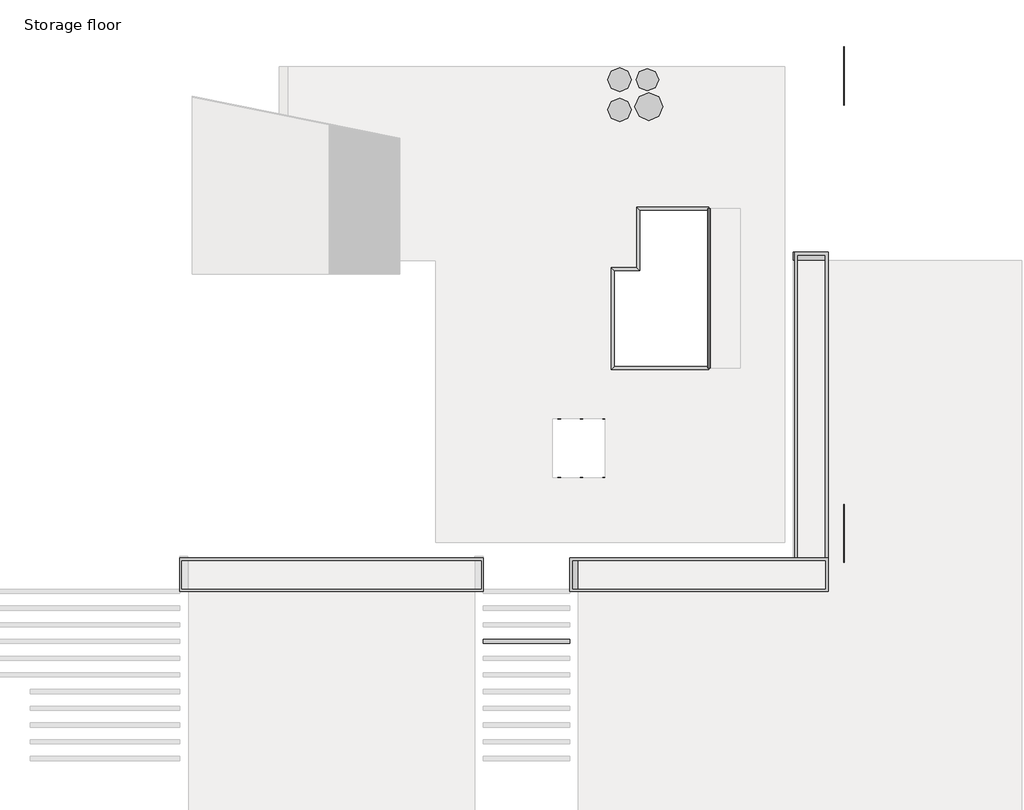
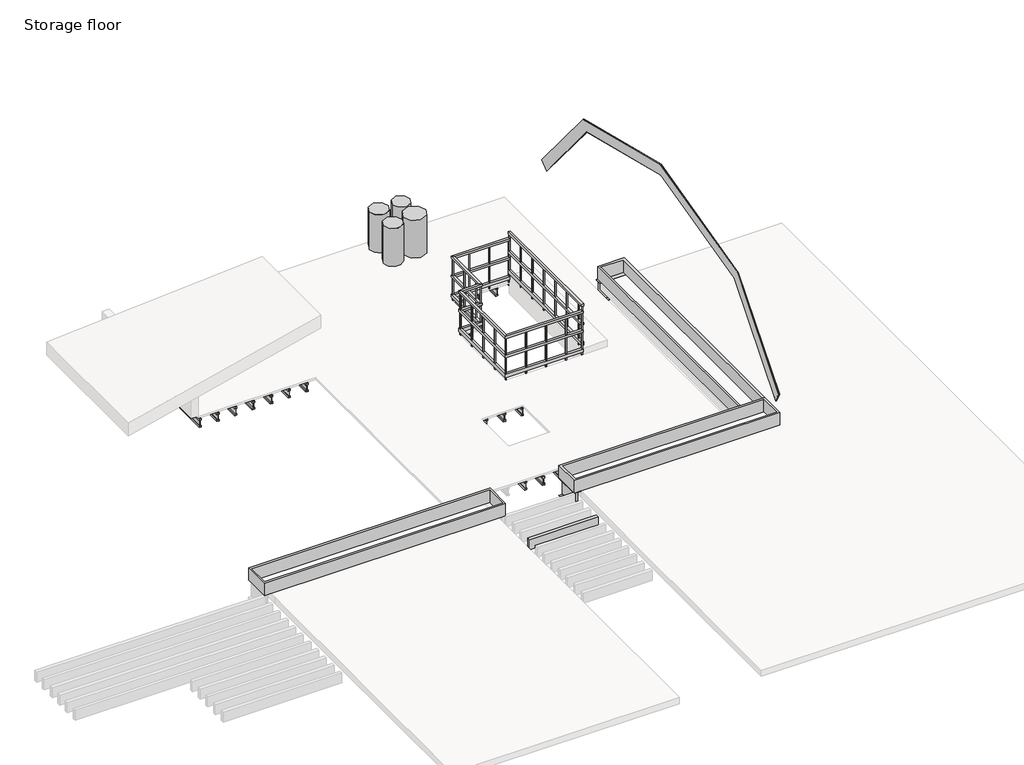
# One storey, part 2 of 2: 29 beams, 9 proxies, 2 railings.
# Revit data of these elements (continued)
# Type "W Shapes : W 6X16 3/4" (continued)
#   Section Area = 7.65 in²
#   Plastic Modulus weak axis = 0.00472801 (stored number, unit not read)
#   Plastic Modulus strong axis = 0.0215278 (stored number, unit not read)
#   Perimeter = 15.0571 m²/m
#   Nominal Weight = 379.441 N/m
#   Moment of Inertia weak axis = 720.08 cm⁴
#   Moment of Inertia strong axis = 8491.12 cm⁴
#   Height = 425.45 mm
#   Flange Thickness = 9.652 mm
#   Elastic Modulus weak axis = 0.00309028 (stored number, unit not read)
#   Elastic Modulus strong axis = 0.0193287 (stored number, unit not read)
#   Centroid Vertical = 212.725 mm
#   Centroid Horizontal = 76.2 mm
#   Length [instance default] = 5' - 0"
#   Structural Material [instance default] = Steel ASTM A992
#   Principal Axes Angle = 0
# Type "W Shapes : W 6X18.5"
#   Section Name Key = "W12x26"
#   Assembly Code = "B10"
#   Width = 152.4 mm
#   Web Thickness = 5.842 mm
#   Web Fillet = 7.62 mm
#   Warping Constant = 163001.3 cm⁶
#   Torsional Moment of Inertia = 12.4869 cm⁴
#   Section Area = 7.65 in²
#   Plastic Modulus weak axis = 0.00472801 (stored number, unit not read)
#   Plastic Modulus strong axis = 0.0215278 (stored number, unit not read)
#   Perimeter = 15.0571 m²/m
#   Nominal Weight = 379.441 N/m
#   Moment of Inertia weak axis = 720.08 cm⁴
#   Moment of Inertia strong axis = 8491.12 cm⁴
#   Height = 469.9 mm
#   Flange Thickness = 9.652 mm
#   Elastic Modulus weak axis = 0.00309028 (stored number, unit not read)
#   Elastic Modulus strong axis = 0.0193287 (stored number, unit not read)
#   Centroid Vertical = 234.95 mm
#   Centroid Horizontal = 76.2 mm
#   Length [instance default] = 5' - 0"
#   Structural Material [instance default] = Steel ASTM A992
#   Principal Axes Angle = 0
# Type "Guardrail - Rectangular 2"
#   Assembly Code = "C2010400"
#   built-in parameter 1008612 = 0.0416667 (stored number, unit not read)
#   built-in parameter 1008611 = 0.0416667 (stored number, unit not read)
#   built-in parameter 1008609 = 0.333333 (stored number, unit not read)
#   built-in parameter 1008604 = 0.166667 (stored number, unit not read)
#   built-in parameter 1008603 = 0.166667 (stored number, unit not read)
#   Railing Height = 3' - 6"
#   built-in parameter 1008630 = 2
#   built-in parameter 1008610 = 1
#   built-in parameter 1008618 = Baluster - Square : 3/4"
# Elements 1, 2, 3, 4, 5, 6, 7, 8, 9, 10, 11, 12, 13, 14, 15, 16, 17, 18, 19, 20, 21, 22, 23, 24, 25, 26 (IfcBeam, "Plywood Web Joist : 2 x 8")
#   Structural Material = Softwood, Lumber
#   Phase Created = New Construction
#   Materials on its faces: "Softwood, Lumber"
# Element 27 (IfcBeam, "Timber : 3x10")
#   Structural Material = Softwood, Lumber
#   Phase Created = New Construction
#   Materials on its faces: "Softwood, Lumber"
# Element 28 (IfcBeam, "W Shapes : W 6X16 3/4")
#   Structural Material = Steel ASTM A992
#   Phase Created = New Construction
#   Materials on its faces: "Steel ASTM A992"
# Element 29 (IfcBeam, "W Shapes : W 6X18.5")
#   Structural Material = Steel ASTM A992
#   Phase Created = New Construction
#   Materials on its faces: "Steel ASTM A992"
# Element 30 (IfcBuildingElementProxy, "Generic Models 2 : Generic Models 1")
#   Phase Created = Existing
# Element 31 (IfcBuildingElementProxy, "Generic Models 4 : Generic Models 1")
#   Phase Created = Existing
# Element 32 (IfcBuildingElementProxy, "Press tank : Press tank")
#   Phase Created = Existing
# Element 33 (IfcBuildingElementProxy, "Press tank1 : Press tank")
#   Phase Created = Existing
# Element 34 (IfcBuildingElementProxy, "Water boiler : Water boiler")
#   Phase Created = Existing
# Element 35 (IfcBuildingElementProxy, "Water boiler1 : Water boiler")
#   Phase Created = Existing
# Element 36 (IfcBuildingElementProxy, "gutter : gutter")
#   Phase Created = New Construction
# Element 37 (IfcBuildingElementProxy, "gutter1 : gutter")
#   Phase Created = New Construction
# Element 38 (IfcBuildingElementProxy, "gutter2 : gutter")
#   Phase Created = New Construction
# Element 39 (IfcRailing, "Guardrail - Rectangular 2")
#   Phase Created = Existing
# Element 40 (IfcRailing, "Guardrail - Rectangular 2")
#   built-in parameter 1008621 = 0.5 (stored number, unit not read)
#   Phase Created = Existing
# Materials
#   "Softwood, Lumber": class "Wood", colour RGB 144 113 62, transparency 0, Description = "Pinus Echinata", Cost = 0
#   "Steel ASTM A992": class "Metal", colour RGB 189 187 185, transparency 0, Description = "Structural steel 50ksi", Cost = 0
